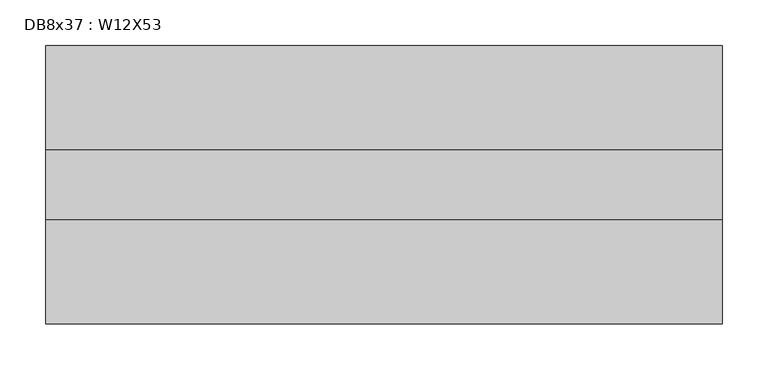
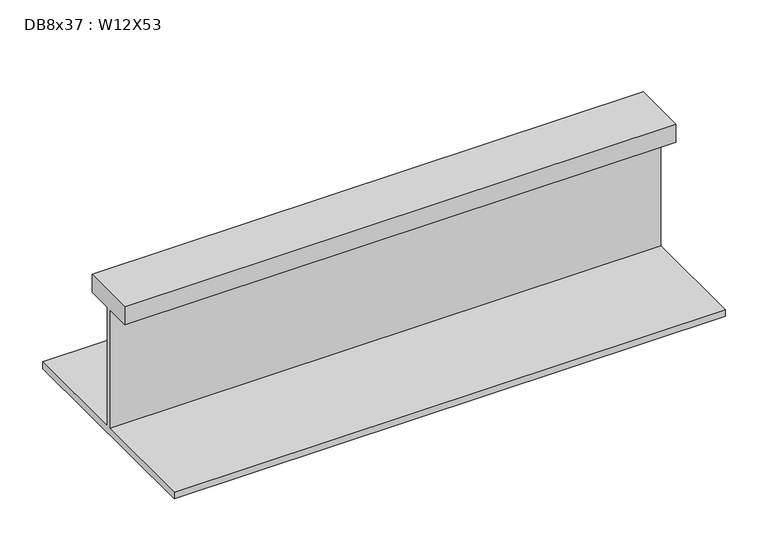
"""IFC4 building model written with IfcOpenShell, lengths in millimetres: beam geometry, DB8x37 : W12X53."""

from ifc_helpers import new_model, si_unit, frame, origin, place, context, project, spatial, polyline, outline, extrude, source, transform, mapped, element, save


def db8x37_w12x53_999e6889(model_context):
    return source(origin(), model_context, "Body", "SweptSolid", [
        extrude(outline(polyline([(38.1, 145.415), (38.1, 120.015), (2.921, 120.015), (2.921, -48.4505), (152.4, -48.4505), (152.4, -58.1025), (-152.4, -58.1025), (-152.4, -48.4505), (-2.921, -48.4505), (-2.921, 120.015), (-38.1, 120.015), (-38.1, 145.415), (38.1, 145.415)])), frame((-355.6, 0.0, 0.0), z_axis=(1.0, 0.0, 0.0), x_axis=(0.0, 1.0, 0.0)), (0.0, 0.0, 1.0), 740.029),
    ])


if __name__ == "__main__":
    model = new_model("IFC4")
    model_context = context("Model", 3, world=origin())
    ifc_project = project(units=[si_unit("LENGTHUNIT", "METRE", prefix="MILLI")], contexts=[model_context])
    site = spatial("IfcSite", under=ifc_project)
    building = spatial("IfcBuilding", under=site)
    placement = place(None, origin())
    db8x37_w12x53_shape = db8x37_w12x53_999e6889(model_context)
    element("IfcBeam", 1, ObjectType="DB8x37 : W12X53", at=placement, inside=building, context=model_context, shape_type="MappedRepresentation", body=[
        mapped(db8x37_w12x53_shape, transform((0.0, 0.0, 0.0), x_axis=(1.0, 0.0, 0.0), y_axis=(0.0, 1.0, 0.0), z_axis=(0.0, 0.0, 1.0))),
    ])
    save(model, "model.ifc")

# Revit data of these elements
# Type "DB8x37 : W12X53"
#   Assembly Code = "B10"
#   W = 53
#   Length [instance default] = 5' - 0"
#   bf = 0' - 10"
#   d = 1' - 0.1"
#   k = 0' - 1 3/8"
#   k2 = 0' - 0.8"
#   tf = 0' - 0.575"
#   tw = 0' - 0.345"
#   A = 0.108333 SF
#   Structural Material [instance default] = Steel ASTM A992
# Element 1 (IfcBeam, "DB8x37 : W12X53")
#   Materials on its faces: "Steel ASTM A992"
# Materials
#   "Steel ASTM A992": class "Metal", colour RGB 199 199 199, transparency 0, Description = "Structural steel 50ksi", Cost = 0
